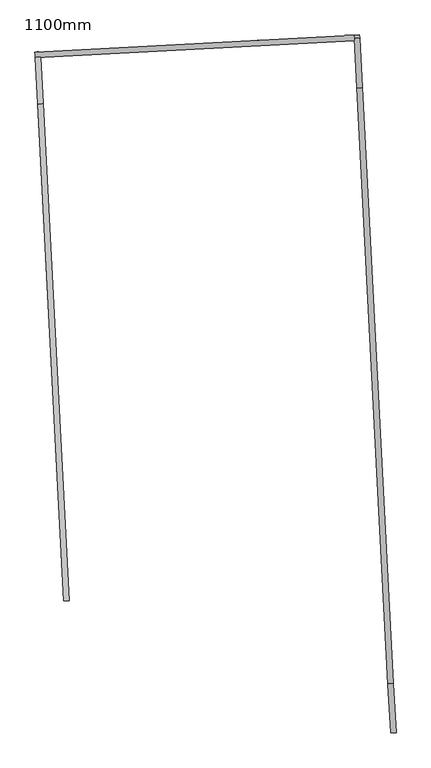
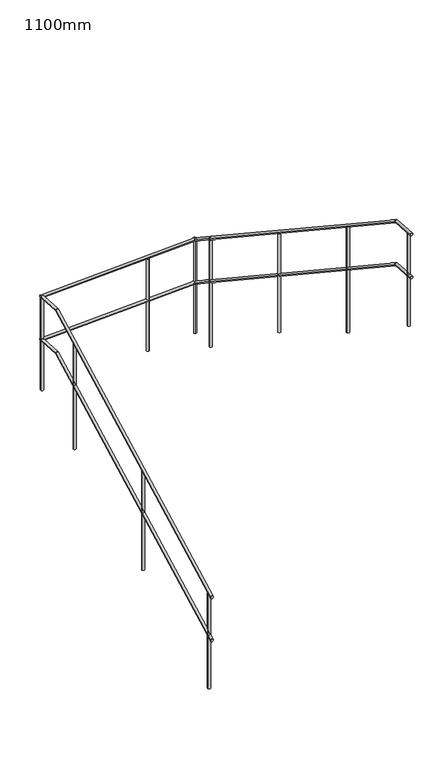
"""IFC4 building model written with IfcOpenShell, lengths in millimetres: railing geometry, 1100mm."""

from ifc_helpers import new_model, si_unit, point, frame, frame_2d, origin, place, context, project, spatial, circle_curve, ellipse_curve, trimmed, segment, composite_curve, outline, extrude, source, transform, mapped, element, save
from ifc_brep_helpers import plane_surface, cylinder_surface, advanced_brep


def railing_1100mm_54c19647(model_context):
    return source(origin(), model_context, "Body", "SolidModel", [
        advanced_brep(
        [(22896.1789103, 12534.7141331, 457.1248327), (22926.1377964, 12536.2842117, 457.1248327), (22754.6396676, 15235.4437699, 2210.0), (22784.5985536, 15237.0138486, 2210.0), (22741.5052252, 15486.0638601, 2210.0), (22771.4641113, 15487.6339388, 2210.0)],
        [
            (0, 1, ellipse_curve(frame((22911.1583533, 12535.4991724, 457.1248327), z_axis=(0.05233595624294174, -0.998629534754574, 0.0), x_axis=(0.0, 0.0, -0.9999999999999999)), 17.8751673, 15.0)),
            (1, 0, ellipse_curve(frame((22911.1583533, 12535.4991724, 457.1248327), z_axis=(0.05233595624294174, -0.998629534754574, 0.0), x_axis=(0.0, 0.0, -0.9999999999999999)), 17.8751673, 15.0)),
            (0, 2),
            (2, 3, ellipse_curve(frame((22769.6191106, 15236.2288092, 2210.0), z_axis=(0.05018733030882238, -0.9576313096148807, -0.28359038545367066), x_axis=(-0.014841974004015643, 0.28320173468646914, -0.9589455111101144)), 15.6421818, 15.0)),
            (3, 1),
            (3, 2, ellipse_curve(frame((22769.6191106, 15236.2288092, 2210.0), z_axis=(0.05018733030882238, -0.9576313096148807, -0.28359038545367066), x_axis=(-0.014841974004015643, 0.28320173468646914, -0.9589455111101144)), 15.6421818, 15.0)),
            (4, 5, circle_curve(frame((22756.4846683, 15486.8488994, 2210.0), z_axis=(-0.05233595624293797, 0.9986295347545743, 0.0), x_axis=(0.9986295347545743, 0.05233595624293797, 0.0)), 15.0)),
            (5, 4, circle_curve(frame((22756.4846683, 15486.8488994, 2210.0), z_axis=(-0.05233595624293797, 0.9986295347545743, 0.0), x_axis=(0.9986295347545743, 0.05233595624293797, 0.0)), 15.0)),
            (2, 4),
            (5, 3),
        ],
        [
            plane_surface(frame((22911.1583533, 12535.4991724, 475.0), z_axis=(0.05233595624294174, -0.998629534754574, 0.0), x_axis=(0.998629534754574, 0.05233595624294174, 0.0))),
            cylinder_surface(frame((22910.731374, 12543.6464234, 462.4127052), z_axis=(0.04391787398555367, -0.8380029565528062, -0.5438954542495689), x_axis=(0.998629534754574, 0.052335956242941746, 0.0)), 15.0),
            plane_surface(frame((22756.4846683, 15486.8488994, 2225.0), z_axis=(-0.05233595624294184, 0.998629534754574, 0.0), x_axis=(0.998629534754574, 0.05233595624294184, 0.0))),
            cylinder_surface(frame((22769.8512715, 15231.7989162, 2210.0), z_axis=(0.05233595624293797, -0.9986295347545743, 0.0), x_axis=(0.9986295347545743, 0.05233595624293797, 0.0)), 15.0),
        ],
        [
            (0, [[1, 2]]),
            (1, [[-1, 3, 4, 5]]),
            (1, [[-2, -5, 6, -3]]),
            (2, [[7, 8]]),
            (3, [[-4, 9, -8, 10]]),
            (3, [[-6, -10, -7, -9]]),
        ],
    ),
        advanced_brep(
        [(22739.9351465, 15516.0227461, 2210.0), (22741.5052252, 15486.0638601, 2210.0), (24475.8528668, 15606.9983388, 2210.0), (24477.4229455, 15577.0394528, 2210.0)],
        [
            (0, 1, circle_curve(frame((22740.7201859, 15501.0433031, 2210.0), z_axis=(-0.998629534754574, -0.05233595624294185, 0.0), x_axis=(0.05233595624294185, -0.998629534754574, 0.0)), 15.0)),
            (1, 0, circle_curve(frame((22740.7201859, 15501.0433031, 2210.0), z_axis=(-0.998629534754574, -0.05233595624294185, 0.0), x_axis=(0.05233595624294185, -0.998629534754574, 0.0)), 15.0)),
            (2, 3, circle_curve(frame((24476.6379061, 15592.0188958, 2210.0), z_axis=(0.998629534754574, 0.05233595624294185, 0.0), x_axis=(0.05233595624294185, -0.998629534754574, 0.0)), 15.0)),
            (3, 2, circle_curve(frame((24476.6379061, 15592.0188958, 2210.0), z_axis=(0.998629534754574, 0.05233595624294185, 0.0), x_axis=(0.05233595624294185, -0.998629534754574, 0.0)), 15.0)),
            (0, 2),
            (3, 1),
        ],
        [
            plane_surface(frame((22740.7201859, 15501.0433031, 2225.0), z_axis=(-0.9986295347545743, -0.052335956242937944, 0.0), x_axis=(0.052335956242937944, -0.9986295347545743, 0.0))),
            plane_surface(frame((24476.6379061, 15592.0188958, 2225.0), z_axis=(0.9986295347545743, 0.052335956242937104, 0.0), x_axis=(0.052335956242937104, -0.9986295347545743, 0.0))),
            cylinder_surface(frame((22740.7201859, 15501.0433031, 2210.0), z_axis=(-0.998629534754574, -0.05233595624294185, 0.0), x_axis=(0.05233595624294185, -0.998629534754574, 0.0)), 15.0),
        ],
        [
            (0, [[1, 2]]),
            (1, [[3, 4]]),
            (2, [[-1, 5, -4, 6]]),
            (2, [[-2, -6, -3, -5]]),
        ],
    ),
        advanced_brep(
        [(24505.8117528, 15608.5684175, 2210.0), (24475.8528668, 15606.9983388, 2210.0), (24506.8498874, 15588.7596297, 2210.0), (24476.8910014, 15587.189551, 2210.0), (24520.7484348, 15323.5595483, 2382.1248327), (24490.7895487, 15321.9894696, 2382.1248327)],
        [
            (0, 1, circle_curve(frame((24490.8323098, 15607.7833782, 2210.0), z_axis=(-0.052335956242937104, 0.9986295347545743, 0.0), x_axis=(-0.9986295347545743, -0.052335956242937104, 0.0)), 15.0)),
            (1, 0, circle_curve(frame((24490.8323098, 15607.7833782, 2210.0), z_axis=(-0.052335956242937104, 0.9986295347545743, 0.0), x_axis=(-0.9986295347545743, -0.052335956242937104, 0.0)), 15.0)),
            (0, 2),
            (2, 3, ellipse_curve(frame((24491.8704444, 15587.9745903, 2210.0), z_axis=(-0.050187330308819895, 0.9576313096148807, -0.28359038545367116), x_axis=(-0.014841974004020982, 0.2832017346864703, 0.9589455111101142)), 15.6421818, 15.0)),
            (3, 1),
            (3, 2, ellipse_curve(frame((24491.8704444, 15587.9745903, 2210.0), z_axis=(-0.050187330308819895, 0.9576313096148807, -0.28359038545367116), x_axis=(-0.014841974004020982, 0.2832017346864703, 0.9589455111101142)), 15.6421818, 15.0)),
            (4, 5, ellipse_curve(frame((24505.7689917, 15322.774509, 2382.1248327), z_axis=(0.052335956242937104, -0.9986295347545743, 0.0), x_axis=(0.0, 0.0, -1.0)), 17.8751673, 15.0)),
            (5, 4, ellipse_curve(frame((24505.7689917, 15322.774509, 2382.1248327), z_axis=(0.052335956242937104, -0.9986295347545743, 0.0), x_axis=(0.0, 0.0, -1.0)), 17.8751673, 15.0)),
            (2, 4),
            (5, 3),
        ],
        [
            plane_surface(frame((24490.8323098, 15607.7833782, 2225.0), z_axis=(-0.05233595624294184, 0.998629534754574, 0.0), x_axis=(0.998629534754574, 0.05233595624294184, 0.0))),
            cylinder_surface(frame((24490.8323098, 15607.7833782, 2210.0), z_axis=(-0.052335956242937104, 0.9986295347545743, 0.0), x_axis=(-0.9986295347545743, -0.052335956242937104, 0.0)), 15.0),
            plane_surface(frame((24505.7689917, 15322.774509, 2400.0), z_axis=(0.052335956242937104, -0.9986295347545743, 0.0), x_axis=(0.9986295347545743, 0.052335956242937104, 0.0))),
            cylinder_surface(frame((24492.0652629, 15584.2572324, 2212.4127052), z_axis=(-0.04391787398554974, 0.8380029565528057, -0.5438954542495701), x_axis=(-0.9986295347545743, -0.0523359562429371, 0.0)), 15.0),
        ],
        [
            (0, [[1, 2]]),
            (1, [[-1, 3, 4, 5]]),
            (1, [[-2, -5, 6, -3]]),
            (2, [[7, 8]]),
            (3, [[-4, 9, -8, 10]]),
            (3, [[-6, -10, -7, -9]]),
        ],
    ),
        advanced_brep(
        [(24520.7484348, 15323.5595483, 2382.1248327), (24490.7895487, 15321.9894696, 2382.1248327), (24690.5490938, 12083.5699627, 4485.0), (24660.5902078, 12081.999884, 4485.0), (24704.4476412, 11818.3698813, 4485.0), (24674.4887551, 11816.7998026, 4485.0)],
        [
            (0, 1, ellipse_curve(frame((24505.7689917, 15322.774509, 2382.1248327), z_axis=(-0.05233595624294191, 0.998629534754574, 0.0), x_axis=(0.0, 0.0, -1.0)), 17.8751673, 15.0)),
            (1, 0, ellipse_curve(frame((24505.7689917, 15322.774509, 2382.1248327), z_axis=(-0.05233595624294191, 0.998629534754574, 0.0), x_axis=(0.0, 0.0, -1.0)), 17.8751673, 15.0)),
            (0, 2),
            (2, 3, ellipse_curve(frame((24675.5696508, 12082.7849234, 4485.0), z_axis=(-0.05018733030882025, 0.9576313096148807, -0.28359038545367127), x_axis=(0.014841974004007963, -0.28320173468647103, -0.9589455111101143)), 15.6421818, 15.0)),
            (3, 1),
            (3, 2, ellipse_curve(frame((24675.5696508, 12082.7849234, 4485.0), z_axis=(-0.05018733030882025, 0.9576313096148807, -0.28359038545367127), x_axis=(0.014841974004007963, -0.28320173468647103, -0.9589455111101143)), 15.6421818, 15.0)),
            (4, 5, circle_curve(frame((24689.4681982, 11817.584842, 4485.0), z_axis=(0.05233595624293375, -0.9986295347545745, 0.0), x_axis=(-0.9986295347545745, -0.05233595624293375, 0.0)), 15.0)),
            (5, 4, circle_curve(frame((24689.4681982, 11817.584842, 4485.0), z_axis=(0.05233595624293375, -0.9986295347545745, 0.0), x_axis=(-0.9986295347545745, -0.05233595624293375, 0.0)), 15.0)),
            (2, 4),
            (5, 3),
        ],
        [
            plane_surface(frame((24505.7689917, 15322.774509, 2400.0), z_axis=(-0.05233595624294191, 0.998629534754574, 0.0), x_axis=(0.998629534754574, 0.05233595624294191, 0.0))),
            cylinder_surface(frame((24506.1959711, 15314.627258, 2387.4127052), z_axis=(-0.04391787398555378, 0.8380029565528053, -0.5438954542495702), x_axis=(-0.998629534754574, -0.052335956242941926, 0.0)), 15.0),
            plane_surface(frame((24689.4681982, 11817.584842, 4500.0), z_axis=(0.05233595624293375, -0.9986295347545745, 0.0), x_axis=(0.9986295347545745, 0.05233595624293375, 0.0))),
            cylinder_surface(frame((24675.33749, 12087.2148164, 4485.0), z_axis=(-0.05233595624293375, 0.9986295347545745, 0.0), x_axis=(-0.9986295347545745, -0.05233595624293375, 0.0)), 15.0),
        ],
        [
            (0, [[1, 2]]),
            (1, [[-1, 3, 4, 5]]),
            (1, [[-2, -5, 6, -3]]),
            (2, [[7, 8]]),
            (3, [[-4, 9, -8, 10]]),
            (3, [[-6, -10, -7, -9]]),
        ],
    ),
        advanced_brep(
        [(22896.1789103, 12534.7141331, 957.1248327), (22926.1377964, 12536.2842117, 957.1248327), (22754.6396676, 15235.4437699, 2710.0), (22784.5985536, 15237.0138486, 2710.0), (22741.5052252, 15486.0638601, 2710.0), (22771.4641113, 15487.6339388, 2710.0)],
        [
            (0, 1, ellipse_curve(frame((22911.1583533, 12535.4991724, 957.1248327), z_axis=(0.05233595624294174, -0.998629534754574, 0.0), x_axis=(0.0, 0.0, -0.9999999999999999)), 17.8751673, 15.0)),
            (1, 0, ellipse_curve(frame((22911.1583533, 12535.4991724, 957.1248327), z_axis=(0.05233595624294174, -0.998629534754574, 0.0), x_axis=(0.0, 0.0, -0.9999999999999999)), 17.8751673, 15.0)),
            (0, 2),
            (2, 3, ellipse_curve(frame((22769.6191106, 15236.2288092, 2710.0), z_axis=(0.05018733030882238, -0.9576313096148807, -0.28359038545367066), x_axis=(-0.014841974004015643, 0.28320173468646914, -0.9589455111101144)), 15.6421818, 15.0)),
            (3, 1),
            (3, 2, ellipse_curve(frame((22769.6191106, 15236.2288092, 2710.0), z_axis=(0.05018733030882238, -0.9576313096148807, -0.28359038545367066), x_axis=(-0.014841974004015643, 0.28320173468646914, -0.9589455111101144)), 15.6421818, 15.0)),
            (4, 5, circle_curve(frame((22756.4846683, 15486.8488994, 2710.0), z_axis=(-0.05233595624293797, 0.9986295347545743, 0.0), x_axis=(0.9986295347545743, 0.05233595624293797, 0.0)), 15.0)),
            (5, 4, circle_curve(frame((22756.4846683, 15486.8488994, 2710.0), z_axis=(-0.05233595624293797, 0.9986295347545743, 0.0), x_axis=(0.9986295347545743, 0.05233595624293797, 0.0)), 15.0)),
            (2, 4),
            (5, 3),
        ],
        [
            plane_surface(frame((22911.1583533, 12535.4991724, 975.0), z_axis=(0.05233595624294174, -0.998629534754574, 0.0), x_axis=(0.998629534754574, 0.05233595624294174, 0.0))),
            cylinder_surface(frame((22910.731374, 12543.6464234, 962.4127052), z_axis=(0.04391787398555367, -0.8380029565528062, -0.5438954542495689), x_axis=(0.998629534754574, 0.052335956242941746, 0.0)), 15.0),
            plane_surface(frame((22756.4846683, 15486.8488994, 2725.0), z_axis=(-0.05233595624294184, 0.998629534754574, 0.0), x_axis=(0.998629534754574, 0.05233595624294184, 0.0))),
            cylinder_surface(frame((22769.8512715, 15231.7989162, 2710.0), z_axis=(0.05233595624293797, -0.9986295347545743, 0.0), x_axis=(0.9986295347545743, 0.05233595624293797, 0.0)), 15.0),
        ],
        [
            (0, [[1, 2]]),
            (1, [[-1, 3, 4, 5]]),
            (1, [[-2, -5, 6, -3]]),
            (2, [[7, 8]]),
            (3, [[-4, 9, -8, 10]]),
            (3, [[-6, -10, -7, -9]]),
        ],
    ),
        advanced_brep(
        [(22739.9351465, 15516.0227461, 2710.0), (22741.5052252, 15486.0638601, 2710.0), (24475.8528668, 15606.9983388, 2710.0), (24477.4229455, 15577.0394528, 2710.0)],
        [
            (0, 1, circle_curve(frame((22740.7201859, 15501.0433031, 2710.0), z_axis=(-0.998629534754574, -0.05233595624294185, 0.0), x_axis=(0.05233595624294185, -0.998629534754574, 0.0)), 15.0)),
            (1, 0, circle_curve(frame((22740.7201859, 15501.0433031, 2710.0), z_axis=(-0.998629534754574, -0.05233595624294185, 0.0), x_axis=(0.05233595624294185, -0.998629534754574, 0.0)), 15.0)),
            (2, 3, circle_curve(frame((24476.6379061, 15592.0188958, 2710.0), z_axis=(0.998629534754574, 0.05233595624294185, 0.0), x_axis=(0.05233595624294185, -0.998629534754574, 0.0)), 15.0)),
            (3, 2, circle_curve(frame((24476.6379061, 15592.0188958, 2710.0), z_axis=(0.998629534754574, 0.05233595624294185, 0.0), x_axis=(0.05233595624294185, -0.998629534754574, 0.0)), 15.0)),
            (0, 2),
            (3, 1),
        ],
        [
            plane_surface(frame((22740.7201859, 15501.0433031, 2725.0), z_axis=(-0.9986295347545743, -0.052335956242937944, 0.0), x_axis=(0.052335956242937944, -0.9986295347545743, 0.0))),
            plane_surface(frame((24476.6379061, 15592.0188958, 2725.0), z_axis=(0.9986295347545743, 0.052335956242937104, 0.0), x_axis=(0.052335956242937104, -0.9986295347545743, 0.0))),
            cylinder_surface(frame((22740.7201859, 15501.0433031, 2710.0), z_axis=(-0.998629534754574, -0.05233595624294185, 0.0), x_axis=(0.05233595624294185, -0.998629534754574, 0.0)), 15.0),
        ],
        [
            (0, [[1, 2]]),
            (1, [[3, 4]]),
            (2, [[-1, 5, -4, 6]]),
            (2, [[-2, -6, -3, -5]]),
        ],
    ),
        advanced_brep(
        [(24505.8117528, 15608.5684175, 2710.0), (24475.8528668, 15606.9983388, 2710.0), (24506.8498874, 15588.7596297, 2710.0), (24476.8910014, 15587.189551, 2710.0), (24520.7484348, 15323.5595483, 2882.1248327), (24490.7895487, 15321.9894696, 2882.1248327)],
        [
            (0, 1, circle_curve(frame((24490.8323098, 15607.7833782, 2710.0), z_axis=(-0.052335956242937104, 0.9986295347545743, 0.0), x_axis=(-0.9986295347545743, -0.052335956242937104, 0.0)), 15.0)),
            (1, 0, circle_curve(frame((24490.8323098, 15607.7833782, 2710.0), z_axis=(-0.052335956242937104, 0.9986295347545743, 0.0), x_axis=(-0.9986295347545743, -0.052335956242937104, 0.0)), 15.0)),
            (0, 2),
            (2, 3, ellipse_curve(frame((24491.8704444, 15587.9745903, 2710.0), z_axis=(-0.050187330308819895, 0.9576313096148807, -0.28359038545367116), x_axis=(-0.014841974004020982, 0.2832017346864703, 0.9589455111101142)), 15.6421818, 15.0)),
            (3, 1),
            (3, 2, ellipse_curve(frame((24491.8704444, 15587.9745903, 2710.0), z_axis=(-0.050187330308819895, 0.9576313096148807, -0.28359038545367116), x_axis=(-0.014841974004020982, 0.2832017346864703, 0.9589455111101142)), 15.6421818, 15.0)),
            (4, 5, ellipse_curve(frame((24505.7689917, 15322.774509, 2882.1248327), z_axis=(0.052335956242937104, -0.9986295347545743, 0.0), x_axis=(0.0, 0.0, -1.0)), 17.8751673, 15.0)),
            (5, 4, ellipse_curve(frame((24505.7689917, 15322.774509, 2882.1248327), z_axis=(0.052335956242937104, -0.9986295347545743, 0.0), x_axis=(0.0, 0.0, -1.0)), 17.8751673, 15.0)),
            (2, 4),
            (5, 3),
        ],
        [
            plane_surface(frame((24490.8323098, 15607.7833782, 2725.0), z_axis=(-0.05233595624294184, 0.998629534754574, 0.0), x_axis=(0.998629534754574, 0.05233595624294184, 0.0))),
            cylinder_surface(frame((24490.8323098, 15607.7833782, 2710.0), z_axis=(-0.052335956242937104, 0.9986295347545743, 0.0), x_axis=(-0.9986295347545743, -0.052335956242937104, 0.0)), 15.0),
            plane_surface(frame((24505.7689917, 15322.774509, 2900.0), z_axis=(0.052335956242937104, -0.9986295347545743, 0.0), x_axis=(0.9986295347545743, 0.052335956242937104, 0.0))),
            cylinder_surface(frame((24492.0652629, 15584.2572324, 2712.4127052), z_axis=(-0.04391787398554974, 0.8380029565528057, -0.5438954542495701), x_axis=(-0.9986295347545743, -0.0523359562429371, 0.0)), 15.0),
        ],
        [
            (0, [[1, 2]]),
            (1, [[-1, 3, 4, 5]]),
            (1, [[-2, -5, 6, -3]]),
            (2, [[7, 8]]),
            (3, [[-4, 9, -8, 10]]),
            (3, [[-6, -10, -7, -9]]),
        ],
    ),
        advanced_brep(
        [(24520.7484348, 15323.5595483, 2882.1248327), (24490.7895487, 15321.9894696, 2882.1248327), (24690.5490938, 12083.5699627, 4985.0), (24660.5902078, 12081.999884, 4985.0), (24704.4476412, 11818.3698813, 4985.0), (24674.4887551, 11816.7998026, 4985.0)],
        [
            (0, 1, ellipse_curve(frame((24505.7689917, 15322.774509, 2882.1248327), z_axis=(-0.05233595624294191, 0.998629534754574, 0.0), x_axis=(0.0, 0.0, -1.0)), 17.8751673, 15.0)),
            (1, 0, ellipse_curve(frame((24505.7689917, 15322.774509, 2882.1248327), z_axis=(-0.05233595624294191, 0.998629534754574, 0.0), x_axis=(0.0, 0.0, -1.0)), 17.8751673, 15.0)),
            (0, 2),
            (2, 3, ellipse_curve(frame((24675.5696508, 12082.7849234, 4985.0), z_axis=(-0.05018733030882025, 0.9576313096148807, -0.28359038545367127), x_axis=(0.014841974004007963, -0.28320173468647103, -0.9589455111101143)), 15.6421818, 15.0)),
            (3, 1),
            (3, 2, ellipse_curve(frame((24675.5696508, 12082.7849234, 4985.0), z_axis=(-0.05018733030882025, 0.9576313096148807, -0.28359038545367127), x_axis=(0.014841974004007963, -0.28320173468647103, -0.9589455111101143)), 15.6421818, 15.0)),
            (4, 5, circle_curve(frame((24689.4681982, 11817.584842, 4985.0), z_axis=(0.05233595624293375, -0.9986295347545745, 0.0), x_axis=(-0.9986295347545745, -0.05233595624293375, 0.0)), 15.0)),
            (5, 4, circle_curve(frame((24689.4681982, 11817.584842, 4985.0), z_axis=(0.05233595624293375, -0.9986295347545745, 0.0), x_axis=(-0.9986295347545745, -0.05233595624293375, 0.0)), 15.0)),
            (2, 4),
            (5, 3),
        ],
        [
            plane_surface(frame((24505.7689917, 15322.774509, 2900.0), z_axis=(-0.05233595624294191, 0.998629534754574, 0.0), x_axis=(0.998629534754574, 0.05233595624294191, 0.0))),
            cylinder_surface(frame((24506.1959711, 15314.627258, 2887.4127052), z_axis=(-0.04391787398555378, 0.8380029565528053, -0.5438954542495702), x_axis=(-0.998629534754574, -0.052335956242941926, 0.0)), 15.0),
            plane_surface(frame((24689.4681982, 11817.584842, 5000.0), z_axis=(0.05233595624293375, -0.9986295347545745, 0.0), x_axis=(0.9986295347545745, 0.05233595624293375, 0.0))),
            cylinder_surface(frame((24675.33749, 12087.2148164, 4985.0), z_axis=(-0.05233595624293375, 0.9986295347545745, 0.0), x_axis=(-0.9986295347545745, -0.05233595624293375, 0.0)), 15.0),
        ],
        [
            (0, [[1, 2]]),
            (1, [[-1, 3, 4, 5]]),
            (1, [[-2, -5, 6, -3]]),
            (2, [[7, 8]]),
            (3, [[-4, 9, -8, 10]]),
            (3, [[-6, -10, -7, -9]]),
        ],
    ),
        extrude(outline(composite_curve([segment(trimmed(circle_curve(frame_2d((24631.3752867, 12926.0636256)), 15.0), [point((24616.3958437, 12925.2785862))], [point((24646.3547297, 12926.8486649))], False, "CARTESIAN"), True, "CONTINUOUS"), segment(trimmed(circle_curve(frame_2d((24631.3752867, 12926.0636256)), 15.0), [point((24646.3547297, 12926.8486649))], [point((24616.3958437, 12925.2785862))], False, "CARTESIAN"), True, "CONTINUOUS")], self_intersect=False)), frame((0.0, 0.0, 3200.0), z_axis=(0.0, 0.0, 1.0), x_axis=(1.0, 0.0, 0.0)), (0.0, 0.0, 1.0), 1225.5555556),
        extrude(outline(composite_curve([segment(trimmed(circle_curve(frame_2d((24568.5721392, 14124.4190673)), 15.0), [point((24553.5926962, 14123.6340279))], [point((24583.5515823, 14125.2041066))], False, "CARTESIAN"), True, "CONTINUOUS"), segment(trimmed(circle_curve(frame_2d((24568.5721392, 14124.4190673)), 15.0), [point((24583.5515823, 14125.2041066))], [point((24553.5926962, 14123.6340279))], False, "CARTESIAN"), True, "CONTINUOUS")], self_intersect=False)), frame((0.0, 0.0, 2500.0), z_axis=(0.0, 0.0, 1.0), x_axis=(1.0, 0.0, 0.0)), (0.0, 0.0, 1.0), 1147.7777778),
        extrude(outline(composite_curve([segment(trimmed(circle_curve(frame_2d((23954.0550706, 15564.6314899)), 15.0), [point((23954.84011, 15549.6520469))], [point((23953.2700313, 15579.6109329))], False, "CARTESIAN"), True, "CONTINUOUS"), segment(trimmed(circle_curve(frame_2d((23954.0550706, 15564.6314899)), 15.0), [point((23953.2700313, 15579.6109329))], [point((23954.84011, 15549.6520469))], False, "CARTESIAN"), True, "CONTINUOUS")], self_intersect=False)), frame((0.0, 0.0, 1625.0), z_axis=(0.0, 0.0, 1.0), x_axis=(1.0, 0.0, 0.0)), (0.0, 0.0, 1.0), 1070.0),
        extrude(outline(composite_curve([segment(trimmed(circle_curve(frame_2d((22785.5520583, 14932.2100558)), 15.0), [point((22800.5315014, 14932.9950952))], [point((22770.5726153, 14931.4250165))], False, "CARTESIAN"), True, "CONTINUOUS"), segment(trimmed(circle_curve(frame_2d((22785.5520583, 14932.2100558)), 15.0), [point((22770.5726153, 14931.4250165))], [point((22800.5315014, 14932.9950952))], False, "CARTESIAN"), True, "CONTINUOUS")], self_intersect=False)), frame((0.0, 0.0, 1275.0), z_axis=(0.0, 0.0, 1.0), x_axis=(1.0, 0.0, 0.0)), (0.0, 0.0, 1.0), 1225.5555556),
        extrude(outline(composite_curve([segment(trimmed(circle_curve(frame_2d((22848.3552058, 13733.8546141)), 15.0), [point((22863.3346489, 13734.6396534))], [point((22833.3757628, 13733.0695748))], False, "CARTESIAN"), True, "CONTINUOUS"), segment(trimmed(circle_curve(frame_2d((22848.3552058, 13733.8546141)), 15.0), [point((22833.3757628, 13733.0695748))], [point((22863.3346489, 13734.6396534))], False, "CARTESIAN"), True, "CONTINUOUS")], self_intersect=False)), frame((0.0, 0.0, 575.0), z_axis=(0.0, 0.0, 1.0), x_axis=(1.0, 0.0, 0.0)), (0.0, 0.0, 1.0), 1147.7777778),
        extrude(outline(composite_curve([segment(trimmed(circle_curve(frame_2d((24505.7689917, 15322.774509)), 15.0), [point((24490.7895487, 15321.9894696))], [point((24520.7484348, 15323.5595483))], False, "CARTESIAN"), True, "CONTINUOUS"), segment(trimmed(circle_curve(frame_2d((24505.7689917, 15322.774509)), 15.0), [point((24520.7484348, 15323.5595483))], [point((24490.7895487, 15321.9894696))], False, "CARTESIAN"), True, "CONTINUOUS")], self_intersect=False)), frame((0.0, 0.0, 1625.0), z_axis=(0.0, 0.0, 1.0), x_axis=(1.0, 0.0, 0.0)), (0.0, 0.0, 1.0), 1245.0),
        extrude(outline(composite_curve([segment(trimmed(circle_curve(frame_2d((24491.6173492, 15592.8039352)), 15.0), [point((24492.4023885, 15577.8244921))], [point((24490.8323098, 15607.7833782))], False, "CARTESIAN"), True, "CONTINUOUS"), segment(trimmed(circle_curve(frame_2d((24491.6173492, 15592.8039352)), 15.0), [point((24490.8323098, 15607.7833782))], [point((24492.4023885, 15577.8244921))], False, "CARTESIAN"), True, "CONTINUOUS")], self_intersect=False)), frame((0.0, 0.0, 1625.0), z_axis=(0.0, 0.0, 1.0), x_axis=(1.0, 0.0, 0.0)), (0.0, 0.0, 1.0), 1070.0),
        extrude(outline(composite_curve([segment(trimmed(circle_curve(frame_2d((22755.6996289, 15501.8283424)), 15.0), [point((22770.6790719, 15502.6133818))], [point((22740.7201859, 15501.0433031))], False, "CARTESIAN"), True, "CONTINUOUS"), segment(trimmed(circle_curve(frame_2d((22755.6996289, 15501.8283424)), 15.0), [point((22740.7201859, 15501.0433031))], [point((22770.6790719, 15502.6133818))], False, "CARTESIAN"), True, "CONTINUOUS")], self_intersect=False)), frame((0.0, 0.0, 1625.0), z_axis=(0.0, 0.0, 1.0), x_axis=(1.0, 0.0, 0.0)), (0.0, 0.0, 1.0), 1070.0),
        extrude(outline(composite_curve([segment(trimmed(circle_curve(frame_2d((24686.8514003, 11867.5163187)), 15.0), [point((24671.8719573, 11866.7312794))], [point((24701.8308434, 11868.3013581))], False, "CARTESIAN"), True, "CONTINUOUS"), segment(trimmed(circle_curve(frame_2d((24686.8514003, 11867.5163187)), 15.0), [point((24701.8308434, 11868.3013581))], [point((24671.8719573, 11866.7312794))], False, "CARTESIAN"), True, "CONTINUOUS")], self_intersect=False)), frame((0.0, 0.0, 3900.0), z_axis=(0.0, 0.0, 1.0), x_axis=(1.0, 0.0, 0.0)), (0.0, 0.0, 1.0), 1070.0),
        extrude(outline(composite_curve([segment(trimmed(circle_curve(frame_2d((22908.5415555, 12585.4306491)), 15.0), [point((22923.5209985, 12586.2156885))], [point((22893.5621125, 12584.6456098))], False, "CARTESIAN"), True, "CONTINUOUS"), segment(trimmed(circle_curve(frame_2d((22908.5415555, 12585.4306491)), 15.0), [point((22893.5621125, 12584.6456098))], [point((22923.5209985, 12586.2156885))], False, "CARTESIAN"), True, "CONTINUOUS")], self_intersect=False)), frame((0.0, 0.0, -125.0), z_axis=(0.0, 0.0, 1.0), x_axis=(1.0, 0.0, 0.0)), (0.0, 0.0, 1.0), 1102.4074074),
    ])


if __name__ == "__main__":
    model = new_model("IFC4")
    model_context = context("Model", 3, world=origin())
    ifc_project = project(units=[si_unit("LENGTHUNIT", "METRE", prefix="MILLI")], contexts=[model_context])
    site = spatial("IfcSite", under=ifc_project)
    building = spatial("IfcBuilding", under=site)
    placement = place(None, origin())
    railing_1100mm_shape = railing_1100mm_54c19647(model_context)
    element("IfcRailing", 1, ObjectType="1100mm", at=placement, inside=building, context=model_context, shape_type="MappedRepresentation", body=[
        mapped(railing_1100mm_shape, transform((0.0, 0.0, 0.0), x_axis=(1.0, 0.0, 0.0), y_axis=(0.0, 1.0, 0.0), z_axis=(0.0, 0.0, 1.0))),
    ])
    save(model, "model.ifc")
